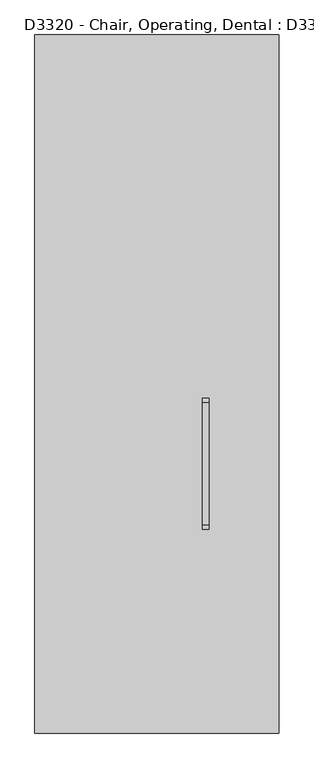
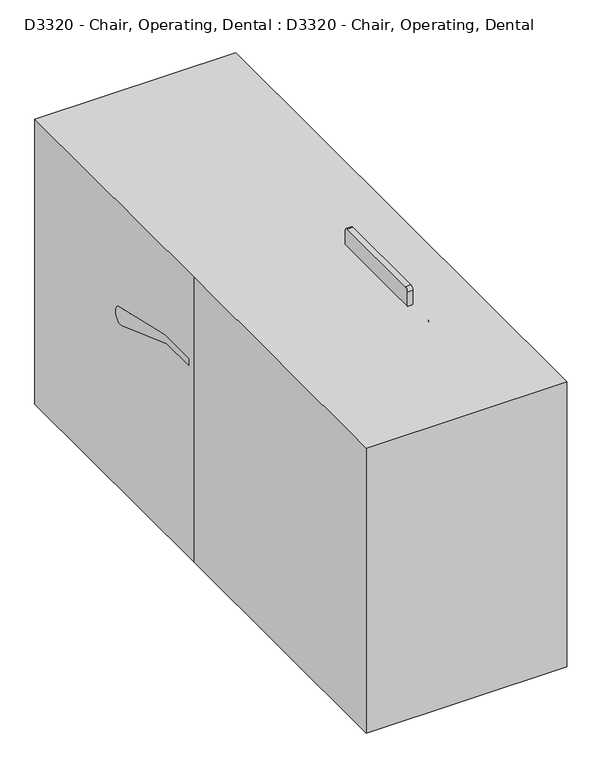
"""IFC4 building model written with IfcOpenShell, lengths in millimetres: proxy geometry, D3320 - Chair, Operating, Dental : D3320 - Chair, Operating, Dental."""

import ifcopenshell
import ifcopenshell.guid

model = None  # the IFC model being written
_history = None  # IfcOwnerHistory: only IFC2X3 demands one
_inside = {}  # id of a spatial element -> (the spatial element, [elements in it])
_under = {}  # id of a project, library or spatial element -> (it, [spatial elements below it])
_declared = {}  # id of a project -> (the project, [libraries it declares])
_typed = {}  # id of a type object -> (the type object, [elements of that type])
_made_of = {}  # id of a material, layer set ... -> (it, [elements and type objects made of it])


def new_model(schema):
    """Start an empty IFC model of exactly this schema.

    Asked for "IFC4X3", IfcOpenShell would pick the latest addendum, in which some entities
    have other attributes; the version numbers below select the first issue.
    IFC2X3 requires an IfcOwnerHistory on every rooted entity: one is made here for all.
    """
    global model, _history
    if schema == "IFC4X3":
        model = ifcopenshell.file(schema_version=(4, 3, 0, 0))
    else:
        model = ifcopenshell.file(schema=schema)
    _inside.clear()
    _under.clear()
    _declared.clear()
    _typed.clear()
    _made_of.clear()
    _history = None
    if model.schema == "IFC2X3":
        org = make("IfcOrganization", Name="unknown")
        user = make(
            "IfcPersonAndOrganization",
            ThePerson=make("IfcPerson", FamilyName="unknown"),
            TheOrganization=org,
        )
        app = make(
            "IfcApplication",
            ApplicationDeveloper=org,
            Version="unknown",
            ApplicationFullName="unknown",
            ApplicationIdentifier="unknown",
        )
        _history = make(
            "IfcOwnerHistory",
            OwningUser=user,
            OwningApplication=app,
            ChangeAction="ADDED",
            CreationDate=0,
        )
    return model


def make(cls, **values):
    """One entity of the class cls with the attributes given. An attribute that is None is left unset."""
    return model.create_entity(
        cls, **{name: value for name, value in values.items() if value is not None}
    )


def rooted(cls, **values):
    """An entity with a GlobalId (a new one), such as an element, a storey or a relation."""
    return make(cls, GlobalId=ifcopenshell.guid.new(), OwnerHistory=_history, **values)


def si_unit(unit_type, name, prefix=None):
    """IfcSIUnit, for example si_unit("LENGTHUNIT", "METRE", prefix="MILLI")."""
    return make("IfcSIUnit", UnitType=unit_type, Prefix=prefix, Name=name)


def assignment(units):
    """IfcUnitAssignment: the units of a project."""
    return None if units is None else make("IfcUnitAssignment", Units=units)


def point(xyz):
    """IfcCartesianPoint."""
    return None if xyz is None else make("IfcCartesianPoint", Coordinates=xyz)


def direction(xyz):
    """IfcDirection."""
    return None if xyz is None else make("IfcDirection", DirectionRatios=xyz)


def frame(location, z_axis=None, x_axis=None):
    """IfcAxis2Placement3D, a coordinate frame: its origin and axes. An axis left out is left unset."""
    return make(
        "IfcAxis2Placement3D",
        Location=point(location),
        Axis=direction(z_axis),
        RefDirection=direction(x_axis),
    )


def frame_2d(location, x_axis=None):
    """IfcAxis2Placement2D, a coordinate frame in the plane: its origin and x axis."""
    return make(
        "IfcAxis2Placement2D", Location=point(location), RefDirection=direction(x_axis)
    )


def origin():
    """The frame at (0, 0, 0) with its axes left unset."""
    return frame((0.0, 0.0, 0.0))


def origin_with_axes():
    """The frame at (0, 0, 0) with the z axis (0, 0, 1) and the x axis (1, 0, 0) written out."""
    return frame((0.0, 0.0, 0.0), z_axis=(0.0, 0.0, 1.0), x_axis=(1.0, 0.0, 0.0))


def place(relative_to, where):
    """IfcLocalPlacement: puts the frame where relative to a parent placement (None: the world)."""
    return make(
        "IfcLocalPlacement", PlacementRelTo=relative_to, RelativePlacement=where
    )


def context(
    kind, dimensions, precision=None, world=None, true_north=None, identifier=None
):
    """IfcGeometricRepresentationContext, for example the 3D "Model" context."""
    return make(
        "IfcGeometricRepresentationContext",
        ContextIdentifier=identifier,
        ContextType=kind,
        CoordinateSpaceDimension=dimensions,
        Precision=precision,
        WorldCoordinateSystem=world,
        TrueNorth=true_north,
    )


def project(units=None, contexts=None):
    """IfcProject with its units and contexts."""
    return rooted(
        "IfcProject",
        Name="project",
        RepresentationContexts=contexts,
        UnitsInContext=assignment(units),
    )


def spatial(cls, under=None, at=None, **own):
    """A site, building, storey or space (cls), placed at a placement, below another one or the project."""
    s = rooted(cls, ObjectPlacement=at, **own)
    if under is not None:
        _under.setdefault(under.id(), (under, []))[1].append(s)
    return s


def polyline(points):
    """IfcPolyline through the points."""
    return make("IfcPolyline", Points=[point(p) for p in points])


def circle_curve(where, radius):
    """IfcCircle in the frame where."""
    return make("IfcCircle", Position=where, Radius=radius)


def ellipse_curve(where, semi_axis1, semi_axis2):
    """IfcEllipse in the frame where."""
    return make(
        "IfcEllipse", Position=where, SemiAxis1=semi_axis1, SemiAxis2=semi_axis2
    )


def trimmed(basis, trim1, trim2, sense, master):
    """IfcTrimmedCurve: the piece of a basis curve between two trims."""
    return make(
        "IfcTrimmedCurve",
        BasisCurve=basis,
        Trim1=trim1,
        Trim2=trim2,
        SenseAgreement=sense,
        MasterRepresentation=master,
    )


def segment(curve, same_sense, transition):
    """IfcCompositeCurveSegment."""
    return make(
        "IfcCompositeCurveSegment",
        Transition=transition,
        SameSense=same_sense,
        ParentCurve=curve,
    )


def composite_curve(segments, self_intersect=None):
    """IfcCompositeCurve: segments joined end to end."""
    return make("IfcCompositeCurve", Segments=segments, SelfIntersect=self_intersect)


def outline(outer, holes=None, kind="AREA"):
    """IfcArbitraryClosedProfileDef: a profile drawn as a closed curve; with holes, ...WithVoids."""
    if holes is None:
        return make("IfcArbitraryClosedProfileDef", ProfileType=kind, OuterCurve=outer)
    return make(
        "IfcArbitraryProfileDefWithVoids",
        ProfileType=kind,
        OuterCurve=outer,
        InnerCurves=holes,
    )


def extrude(swept, where, along, depth):
    """IfcExtrudedAreaSolid: the profile swept, set in the frame where, extruded along a direction by depth."""
    return make(
        "IfcExtrudedAreaSolid",
        SweptArea=swept,
        Position=where,
        ExtrudedDirection=direction(along),
        Depth=depth,
    )


def shape(context_of_items, identifier, shape_type, items):
    """IfcShapeRepresentation: the items that make up one representation, for example the "Body"."""
    return make(
        "IfcShapeRepresentation",
        ContextOfItems=context_of_items,
        RepresentationIdentifier=identifier,
        RepresentationType=shape_type,
        Items=items,
    )


def source(mapping_origin, context_of_items, identifier, shape_type, items):
    """IfcRepresentationMap: a shape defined once, which mapped items show again and again."""
    return make(
        "IfcRepresentationMap",
        MappingOrigin=mapping_origin,
        MappedRepresentation=shape(context_of_items, identifier, shape_type, items),
    )


def transform(
    local_origin,
    x_axis=None,
    y_axis=None,
    z_axis=None,
    scale=None,
    scale2=None,
    scale3=None,
    uniform=True,
):
    """IfcCartesianTransformationOperator3D, or its non-uniform kind. x_axis, y_axis, z_axis: its Axis1, 2, 3."""
    if uniform:
        return make(
            "IfcCartesianTransformationOperator3D",
            Axis1=direction(x_axis),
            Axis2=direction(y_axis),
            LocalOrigin=point(local_origin),
            Scale=scale,
            Axis3=direction(z_axis),
        )
    return make(
        "IfcCartesianTransformationOperator3DnonUniform",
        Axis1=direction(x_axis),
        Axis2=direction(y_axis),
        LocalOrigin=point(local_origin),
        Scale=scale,
        Axis3=direction(z_axis),
        Scale2=scale2,
        Scale3=scale3,
    )


def mapped(mapping_source, mapping_target):
    """IfcMappedItem: shows the shape of a source again, moved by a transform."""
    return make(
        "IfcMappedItem", MappingSource=mapping_source, MappingTarget=mapping_target
    )


def made_of(thing, what):
    """Note that an element or type object is made of a material, layer set ...; save() writes the relation."""
    if what is not None:
        _made_of.setdefault(what.id(), (what, []))[1].append(thing)
    return thing


def element(
    cls,
    number,
    at=None,
    inside=None,
    cuts=None,
    type_object=None,
    material=None,
    context=None,
    identifier="Body",
    shape_type=None,
    held_by="IfcProductDefinitionShape",
    body=None,
    shapes=None,
    **own,
):
    """One element of the class cls, such as IfcWall. Its Tag is "e" and its number.

    at: its placement. inside: the storey or other place that contains it. cuts: it is an
    opening in that element (IfcRelVoidsElement). A single representation is given by context,
    identifier, shape_type and body (its items); several are given by shapes. held_by: the class
    of the entity that holds the representations. save() writes the other relations.
    """
    e = rooted(cls, Tag="e%d" % number, ObjectPlacement=at, **own)
    if body is not None:
        shapes = [shape(context, identifier, shape_type, body)]
    if shapes is not None:
        e.Representation = make(held_by, Representations=shapes)
    if inside is not None:
        _inside.setdefault(inside.id(), (inside, []))[1].append(e)
    if cuts is not None:
        rooted(
            "IfcRelVoidsElement", RelatingBuildingElement=cuts, RelatedOpeningElement=e
        )
    if type_object is not None:
        _typed.setdefault(type_object.id(), (type_object, []))[1].append(e)
    return made_of(e, material)


def aggregate(whole, parts):
    """IfcRelAggregates: a whole, such as a stair, and the parts it consists of."""
    return rooted("IfcRelAggregates", RelatingObject=whole, RelatedObjects=parts)


def save(model, path):
    """Write the relations noted so far, then the file.

    IfcRelAggregates (storeys below a building ...), IfcRelContainedInSpatialStructure (elements
    in a storey), IfcRelDefinesByType, IfcRelAssociatesMaterial and IfcRelDeclares: one each for
    every whole, place, type object, material and project.
    """
    for whole, parts in _under.values():
        aggregate(whole, parts)
    for where, things in _inside.values():
        rooted(
            "IfcRelContainedInSpatialStructure",
            RelatedElements=things,
            RelatingStructure=where,
        )
    for kind, things in _typed.values():
        rooted("IfcRelDefinesByType", RelatedObjects=things, RelatingType=kind)
    for what, things in _made_of.values():
        rooted("IfcRelAssociatesMaterial", RelatedObjects=things, RelatingMaterial=what)
    for by, libraries in _declared.values():
        rooted("IfcRelDeclares", RelatingContext=by, RelatedDefinitions=libraries)
    model.write(path)


def plane_surface(at):
    """IfcPlane: the flat surface through the origin of the frame at, square to its z axis."""
    return make("IfcPlane", Position=at)


def cylinder_surface(at, radius):
    """IfcCylindricalSurface: all points at the distance radius from the z axis of the frame at."""
    return make("IfcCylindricalSurface", Position=at, Radius=radius)


def revolved_surface(curve, axis_point, axis_direction):
    """IfcSurfaceOfRevolution: the curve turned about the line through axis_point along axis_direction."""
    return make(
        "IfcSurfaceOfRevolution",
        SweptCurve=make("IfcArbitraryOpenProfileDef", ProfileType="CURVE", Curve=curve),
        AxisPosition=make("IfcAxis1Placement", Location=point(axis_point), Axis=direction(axis_direction)),
    )


def spline_surface(u_degree, v_degree, points, u_multiplicities, v_multiplicities, u_knots, v_knots, weights=None):
    """IfcBSplineSurfaceWithKnots; with weights, IfcRationalBSplineSurfaceWithKnots. points: one row for each step in u."""
    own = dict(
        UDegree=u_degree,
        VDegree=v_degree,
        ControlPointsList=[[point(p) for p in row] for row in points],
        SurfaceForm="UNSPECIFIED",
        UClosed=False,
        VClosed=False,
        SelfIntersect=False,
        UMultiplicities=u_multiplicities,
        VMultiplicities=v_multiplicities,
        UKnots=u_knots,
        VKnots=v_knots,
        KnotSpec="UNSPECIFIED",
    )
    if weights is None:
        return make("IfcBSplineSurfaceWithKnots", **own)
    return make("IfcRationalBSplineSurfaceWithKnots", WeightsData=weights, **own)


def advanced_brep(points, edges, surfaces, faces):
    """IfcAdvancedBrep: a solid bounded by faces that lie on surfaces and meet in shared edges.

    An edge is (start, end): straight between two places in points (the first is 0);
    or (start, end, curve); or (start, end, curve, False) where it runs against its curve.
    A face is (place in surfaces, loops), or (place, loops, False) where it looks against
    its surface's normal. A loop lists edges by number (the first is 1), with a minus sign
    where the edge is run from its end to its start. The first loop is the outer one.
    """
    corners = [point(p) for p in points]
    vertices = [make("IfcVertexPoint", VertexGeometry=c) for c in corners]
    made = []
    for start, end, *more in edges:
        made.append(
            make(
                "IfcEdgeCurve",
                EdgeStart=vertices[start],
                EdgeEnd=vertices[end],
                EdgeGeometry=more[0] if more else make("IfcPolyline", Points=[corners[start], corners[end]]),
                SameSense=more[1] if len(more) > 1 else True,
            )
        )
    hull = []
    for where, loops, *sense in faces:
        bounds = []
        for j, loop in enumerate(loops):
            ring = [make("IfcOrientedEdge", EdgeElement=made[abs(k) - 1], Orientation=k > 0) for k in loop]
            bounds.append(
                make(
                    "IfcFaceOuterBound" if j == 0 else "IfcFaceBound",
                    Bound=make("IfcEdgeLoop", EdgeList=ring),
                    Orientation=True,
                )
            )
        hull.append(make("IfcAdvancedFace", Bounds=bounds, FaceSurface=surfaces[where], SameSense=sense[0] if sense else True))
    return make("IfcAdvancedBrep", Outer=make("IfcClosedShell", CfsFaces=hull))


def d3320_chair_operating_dental_d3320_chair_operating_dental_678bfee4(model_context):
    return source(origin(), model_context, "Body", "SolidModel", [
        advanced_brep(
        [(330.2, -282.0868489, 807.4979758), (330.2, -282.0868489, 845.5979758), (330.2, -212.2368489, 877.3479758), (330.2, -250.3368489, 877.3479758)],
        [
            (0, 1, circle_curve(frame((330.2, -282.0868489, 826.5479758), z_axis=(0.0, -1.0, 0.0), x_axis=(0.0, 0.0, 1.0)), 19.05)),
            (1, 0, circle_curve(frame((330.2, -282.0868489, 826.5479758), z_axis=(0.0, -1.0, 0.0), x_axis=(0.0, 0.0, 1.0)), 19.05)),
            (2, 3, circle_curve(frame((330.2, -231.2868489, 877.3479758), z_axis=(0.0, 0.0, 1.0), x_axis=(0.0, -1.0, 0.0)), 19.05)),
            (3, 2, circle_curve(frame((330.2, -231.2868489, 877.3479758), z_axis=(0.0, 0.0, 1.0), x_axis=(0.0, -1.0, 0.0)), 19.05)),
            (3, 1, circle_curve(frame((330.2, -282.0868489, 877.3479758), z_axis=(-1.0, 0.0, 0.0), x_axis=(0.0, 0.0, -1.0)), 31.75)),
            (0, 2, circle_curve(frame((330.2, -282.0868489, 877.3479758), z_axis=(1.0, 0.0, 0.0), x_axis=(0.0, 0.0, -1.0)), 69.85)),
        ],
        [
            plane_surface(frame((330.2, -282.0868489, 826.5479758), z_axis=(0.0, -1.0, 0.0), x_axis=(1.0, 0.0, 0.0))),
            plane_surface(frame((330.2, -231.2868489, 877.3479758), z_axis=(0.0, 0.0, 1.0), x_axis=(1.0, 0.0, 0.0))),
            revolved_surface(trimmed(ellipse_curve(frame((330.2, -282.0868489, 826.5479758), z_axis=(0.0, -1.0, 0.0), x_axis=(0.0, 0.0, 1.0)), 19.05, 19.05), [point((330.2, -282.0868489, 807.4979758))], [point((330.2, -282.0868489, 845.5979758))], True, "CARTESIAN"), (330.2, -282.0868489, 877.3479758), (1.0, 0.0, 0.0)),
            revolved_surface(trimmed(ellipse_curve(frame((330.2, -282.0868489, 826.5479758), z_axis=(0.0, -1.0, 0.0), x_axis=(0.0, 0.0, 1.0)), 19.05, 19.05), [point((330.2, -282.0868489, 845.5979758))], [point((330.2, -282.0868489, 807.4979758))], True, "CARTESIAN"), (330.2, -282.0868489, 877.3479758), (1.0, 0.0, 0.0)),
        ],
        [
            (0, [[1, 2]]),
            (1, [[3, 4]]),
            (2, [[5, -1, 6, -4]]),
            (3, [[-6, -2, -5, -3]]),
        ],
    ),
        extrude(outline(composite_curve([segment(trimmed(circle_curve(frame_2d((826.5479758, 330.2)), 19.05), [point((807.4979758, 330.2))], [point((845.5979758, 330.2))], False, "CARTESIAN"), True, "CONTINUOUS"), segment(trimmed(circle_curve(frame_2d((826.5479758, 330.2)), 19.05), [point((845.5979758, 330.2))], [point((807.4979758, 330.2))], False, "CARTESIAN"), True, "CONTINUOUS")], self_intersect=False)), frame((0.0, -629.7082464, 0.0), z_axis=(0.0, 1.0, 0.0), x_axis=(0.0, 0.0, 1.0)), (0.0, 0.0, 1.0), 347.6213974),
        advanced_brep(
        [(330.2, -629.7082464, 845.5979758), (330.2, -629.7082464, 807.4979758), (330.2, -699.5582464, 775.7479758), (330.2, -661.4582464, 775.7479758)],
        [
            (0, 1, circle_curve(frame((330.2, -629.7082464, 826.5479758), z_axis=(0.0, 1.0, 0.0), x_axis=(0.0, 0.0, -1.0)), 19.05)),
            (1, 0, circle_curve(frame((330.2, -629.7082464, 826.5479758), z_axis=(0.0, 1.0, 0.0), x_axis=(0.0, 0.0, -1.0)), 19.05)),
            (2, 3, circle_curve(frame((330.2, -680.5082464, 775.7479758), z_axis=(0.0, 0.0, -1.0), x_axis=(0.0, 1.0, 0.0)), 19.05)),
            (3, 2, circle_curve(frame((330.2, -680.5082464, 775.7479758), z_axis=(0.0, 0.0, -1.0), x_axis=(0.0, 1.0, 0.0)), 19.05)),
            (3, 1, circle_curve(frame((330.2, -629.7082464, 775.7479758), z_axis=(-1.0, 0.0, 0.0), x_axis=(0.0, 0.0, 1.0)), 31.75)),
            (0, 2, circle_curve(frame((330.2, -629.7082464, 775.7479758), z_axis=(1.0, 0.0, 0.0), x_axis=(0.0, 0.0, 1.0)), 69.85)),
        ],
        [
            plane_surface(frame((330.2, -629.7082464, 826.5479758), z_axis=(0.0, 1.0, 0.0), x_axis=(1.0, 0.0, 0.0))),
            plane_surface(frame((330.2, -680.5082464, 775.7479758), z_axis=(0.0, 0.0, -1.0), x_axis=(1.0, 0.0, 0.0))),
            revolved_surface(trimmed(ellipse_curve(frame((330.2, -629.7082464, 826.5479758), z_axis=(0.0, 1.0, 0.0), x_axis=(0.0, 0.0, -1.0)), 19.05, 19.05), [point((330.2, -629.7082464, 845.5979758))], [point((330.2, -629.7082464, 807.4979758))], True, "CARTESIAN"), (330.2, -629.7082464, 775.7479758), (1.0, 0.0, 0.0)),
            revolved_surface(trimmed(ellipse_curve(frame((330.2, -629.7082464, 826.5479758), z_axis=(0.0, 1.0, 0.0), x_axis=(0.0, 0.0, -1.0)), 19.05, 19.05), [point((330.2, -629.7082464, 807.4979758))], [point((330.2, -629.7082464, 845.5979758))], True, "CARTESIAN"), (330.2, -629.7082464, 775.7479758), (1.0, 0.0, 0.0)),
        ],
        [
            (0, [[1, 2]]),
            (1, [[3, 4]]),
            (2, [[5, -1, 6, -4]]),
            (3, [[-6, -2, -5, -3]]),
        ],
    ),
        extrude(outline(composite_curve([segment(polyline([(-54.312137, 904.4198133), (-409.912137, 904.4198133)]), True, "CONTINUOUS"), segment(trimmed(circle_curve(frame_2d((-409.912137, 917.1198133)), 12.7), [point((-409.912137, 904.4198133))], [point((-422.612137, 917.1198133))], False, "CARTESIAN"), True, "CONTINUOUS"), segment(polyline([(-422.612137, 917.1198133), (-422.612137, 1120.3198133)]), True, "CONTINUOUS"), segment(trimmed(circle_curve(frame_2d((-409.912137, 1120.3198133)), 12.7), [point((-422.612137, 1120.3198133))], [point((-409.912137, 1133.0198133))], False, "CARTESIAN"), True, "CONTINUOUS"), segment(polyline([(-409.912137, 1133.0198133), (-54.312137, 1133.0198133)]), True, "CONTINUOUS"), segment(trimmed(circle_curve(frame_2d((-54.312137, 1120.3198133)), 12.7), [point((-54.312137, 1133.0198133))], [point((-41.612137, 1120.3198133))], False, "CARTESIAN"), True, "CONTINUOUS"), segment(polyline([(-41.612137, 1120.3198133), (-41.612137, 917.1198133)]), True, "CONTINUOUS"), segment(trimmed(circle_curve(frame_2d((-54.312137, 917.1198133)), 12.7), [point((-41.612137, 917.1198133))], [point((-54.312137, 904.4198133))], False, "CARTESIAN"), True, "CONTINUOUS")], self_intersect=False)), frame((133.35, 0.0, 0.0), z_axis=(1.0, 0.0, 0.0), x_axis=(0.0, 1.0, 0.0)), (0.0, 0.0, 1.0), 19.05),
        advanced_brep(
        [(152.4, -231.2868489, 909.123847), (152.4, -231.2868489, 947.223847), (279.4, -231.2868489, 947.223847), (279.4, -231.2868489, 909.123847), (311.15, -231.2868489, 877.373847), (349.25, -231.2868489, 877.373847)],
        [
            (0, 1, circle_curve(frame((152.4, -231.2868489, 928.173847), z_axis=(-1.0, 0.0, 0.0), x_axis=(0.0, 0.0, 1.0)), 19.05)),
            (1, 0, circle_curve(frame((152.4, -231.2868489, 928.173847), z_axis=(-1.0, 0.0, 0.0), x_axis=(0.0, 0.0, 1.0)), 19.05)),
            (1, 2),
            (2, 3, circle_curve(frame((279.4, -231.2868489, 928.173847), z_axis=(-1.0, 0.0, 0.0), x_axis=(0.0, 0.0, 1.0)), 19.05)),
            (3, 0),
            (3, 2, circle_curve(frame((279.4, -231.2868489, 928.173847), z_axis=(-1.0, 0.0, 0.0), x_axis=(0.0, 0.0, 1.0)), 19.05)),
            (4, 5, circle_curve(frame((330.2, -231.2868489, 877.373847), z_axis=(0.0, 0.0, -1.0), x_axis=(1.0, 0.0, 0.0)), 19.05)),
            (5, 4, circle_curve(frame((330.2, -231.2868489, 877.373847), z_axis=(0.0, 0.0, -1.0), x_axis=(1.0, 0.0, 0.0)), 19.05)),
            (4, 3, circle_curve(frame((279.4, -231.2868489, 877.373847), z_axis=(0.0, -1.0, 0.0), x_axis=(0.0, 0.0, 1.0)), 31.75)),
            (2, 5, circle_curve(frame((279.4, -231.2868489, 877.373847), z_axis=(0.0, 1.0, 0.0), x_axis=(0.0, 0.0, 1.0)), 69.85)),
        ],
        [
            plane_surface(frame((152.4, -231.2868489, 928.173847), z_axis=(-1.0, 0.0, 0.0), x_axis=(0.0, -1.0, 0.0))),
            cylinder_surface(frame((152.4, -231.2868489, 928.173847), z_axis=(-1.0, 0.0, 0.0), x_axis=(0.0, 0.0, 1.0)), 19.05),
            plane_surface(frame((330.2, -231.2868489, 877.373847), z_axis=(0.0, 0.0, -1.0), x_axis=(0.0, -1.0, 0.0))),
            revolved_surface(trimmed(ellipse_curve(frame((279.4, -231.2868489, 928.173847), z_axis=(-1.0, 0.0, 0.0), x_axis=(0.0, 0.0, 1.0)), 19.05, 19.05), [point((279.4, -231.2868489, 947.223847))], [point((279.4, -231.2868489, 909.123847))], True, "CARTESIAN"), (279.4, -231.2868489, 877.373847), (0.0, 1.0, 0.0)),
            revolved_surface(trimmed(ellipse_curve(frame((279.4, -231.2868489, 928.173847), z_axis=(-1.0, 0.0, 0.0), x_axis=(0.0, 0.0, 1.0)), 19.05, 19.05), [point((279.4, -231.2868489, 909.123847))], [point((279.4, -231.2868489, 947.223847))], True, "CARTESIAN"), (279.4, -231.2868489, 877.373847), (0.0, 1.0, 0.0)),
        ],
        [
            (0, [[1, 2]]),
            (1, [[-2, 3, 4, 5]]),
            (1, [[-1, -5, 6, -3]]),
            (2, [[7, 8]]),
            (3, [[9, -4, 10, -7]]),
            (4, [[-10, -6, -9, -8]]),
        ],
    ),
        advanced_brep(
        [(152.4, -680.5082464, 147.0979758), (152.4, -680.5082464, 185.1979758), (279.4, -680.5082464, 147.0979758), (279.4, -680.5082464, 185.1979758), (349.25, -680.5082464, 216.9479758), (311.15, -680.5082464, 216.9479758)],
        [
            (0, 1, circle_curve(frame((152.4, -680.5082464, 166.1479758), z_axis=(-1.0, 0.0, 0.0), x_axis=(0.0, 0.0, 1.0)), 19.05)),
            (1, 0, circle_curve(frame((152.4, -680.5082464, 166.1479758), z_axis=(-1.0, 0.0, 0.0), x_axis=(0.0, 0.0, 1.0)), 19.05)),
            (0, 2),
            (2, 3, circle_curve(frame((279.4, -680.5082464, 166.1479758), z_axis=(-1.0, 0.0, 0.0), x_axis=(0.0, 0.0, 1.0)), 19.05)),
            (3, 1),
            (3, 2, circle_curve(frame((279.4, -680.5082464, 166.1479758), z_axis=(-1.0, 0.0, 0.0), x_axis=(0.0, 0.0, 1.0)), 19.05)),
            (4, 5, circle_curve(frame((330.2, -680.5082464, 216.9479758), z_axis=(0.0, 0.0, 1.0), x_axis=(-1.0, 0.0, 0.0)), 19.05)),
            (5, 4, circle_curve(frame((330.2, -680.5082464, 216.9479758), z_axis=(0.0, 0.0, 1.0), x_axis=(-1.0, 0.0, 0.0)), 19.05)),
            (5, 3, circle_curve(frame((279.4, -680.5082464, 216.9479758), z_axis=(0.0, 1.0, 0.0), x_axis=(0.0, 0.0, -1.0)), 31.75)),
            (2, 4, circle_curve(frame((279.4, -680.5082464, 216.9479758), z_axis=(0.0, -1.0, 0.0), x_axis=(0.0, 0.0, -1.0)), 69.85)),
        ],
        [
            plane_surface(frame((152.4, -680.5082464, 166.1479758), z_axis=(-1.0, 0.0, 0.0), x_axis=(0.0, -1.0, 0.0))),
            cylinder_surface(frame((152.4, -680.5082464, 166.1479758), z_axis=(-1.0, 0.0, 0.0), x_axis=(0.0, 0.0, 1.0)), 19.05),
            plane_surface(frame((330.2, -680.5082464, 216.9479758), z_axis=(0.0, 0.0, 1.0), x_axis=(0.0, -1.0, 0.0))),
            revolved_surface(trimmed(ellipse_curve(frame((279.4, -680.5082464, 166.1479758), z_axis=(-1.0, 0.0, 0.0), x_axis=(0.0, 0.0, 1.0)), 19.05, 19.05), [point((279.4, -680.5082464, 147.0979758))], [point((279.4, -680.5082464, 185.1979758))], True, "CARTESIAN"), (279.4, -680.5082464, 216.9479758), (0.0, -1.0, 0.0)),
            revolved_surface(trimmed(ellipse_curve(frame((279.4, -680.5082464, 166.1479758), z_axis=(-1.0, 0.0, 0.0), x_axis=(0.0, 0.0, 1.0)), 19.05, 19.05), [point((279.4, -680.5082464, 185.1979758))], [point((279.4, -680.5082464, 147.0979758))], True, "CARTESIAN"), (279.4, -680.5082464, 216.9479758), (0.0, -1.0, 0.0)),
        ],
        [
            (0, [[1, 2]]),
            (1, [[-1, 3, 4, 5]]),
            (1, [[-2, -5, 6, -3]]),
            (2, [[7, 8]]),
            (3, [[9, -4, 10, -8]]),
            (4, [[-10, -6, -9, -7]]),
        ],
    ),
        extrude(outline(composite_curve([segment(trimmed(circle_curve(frame_2d((493.8256126, 645.6714008)), 19.05), [point((474.7756126, 645.6714008))], [point((512.8756126, 645.6714008))], False, "CARTESIAN"), True, "CONTINUOUS"), segment(trimmed(circle_curve(frame_2d((493.8256126, 645.6714008)), 19.05), [point((512.8756126, 645.6714008))], [point((474.7756126, 645.6714008))], False, "CARTESIAN"), True, "CONTINUOUS")], self_intersect=False)), frame((-306.1189765, 0.0, 0.0), z_axis=(1.0, 0.0, 0.0), x_axis=(0.0, 1.0, 0.0)), (0.0, 0.0, 1.0), 610.9189765),
        extrude(outline(composite_curve([segment(trimmed(circle_curve(frame_2d((330.2, -680.5082464)), 19.05), [point((349.25, -680.5082464))], [point((311.15, -680.5082464))], False, "CARTESIAN"), True, "CONTINUOUS"), segment(trimmed(circle_curve(frame_2d((330.2, -680.5082464)), 19.05), [point((311.15, -680.5082464))], [point((349.25, -680.5082464))], False, "CARTESIAN"), True, "CONTINUOUS")], self_intersect=False)), frame((0.0, 0.0, 216.9479758), z_axis=(0.0, 0.0, 1.0), x_axis=(1.0, 0.0, 0.0)), (0.0, 0.0, 1.0), 558.8),
        extrude(outline(composite_curve([segment(trimmed(circle_curve(frame_2d((208.2843617, -50.8)), 50.8), [point((208.2843617, 0.0))], [point((243.3133982, -14.0086069))], False, "CARTESIAN"), True, "CONTINUOUS"), segment(polyline([(243.3133982, -14.0086069), (332.2133982, -167.9879237)]), True, "CONTINUOUS"), segment(trimmed(circle_curve(frame_2d((16.6967808, -350.1515277)), 364.327208), [point((332.2133982, -167.9879237))], [point((381.0, -345.9707394))], False, "CARTESIAN"), True, "CONTINUOUS"), segment(polyline([(381.0, -345.9707394), (381.0, -422.1707394)]), True, "CONTINUOUS"), segment(trimmed(circle_curve(frame_2d((182.0559291, -422.1707394)), 198.9440709), [point((381.0, -422.1707394))], [point((309.9347128, -574.5707394))], False, "CARTESIAN"), True, "CONTINUOUS"), segment(polyline([(309.9347128, -574.5707394), (-50.8, -574.5707394)]), True, "CONTINUOUS"), segment(trimmed(circle_curve(frame_2d((22.4448791, -442.6982999)), 150.8481111), [point((-50.8, -574.5707394))], [point((-127.0, -422.1707394))], False, "CARTESIAN"), True, "CONTINUOUS"), segment(polyline([(-127.0, -422.1707394), (-127.0, -345.9707394)]), True, "CONTINUOUS"), segment(trimmed(circle_curve(frame_2d((237.3032191, -350.1515277)), 364.327208), [point((-127.0, -345.9707394))], [point((-78.2133983, -167.9879237))], False, "CARTESIAN"), True, "CONTINUOUS"), segment(polyline([(-78.2133983, -167.9879237), (10.6866017, -14.0086069)]), True, "CONTINUOUS"), segment(trimmed(circle_curve(frame_2d((45.7156382, -50.8)), 50.8), [point((10.6866017, -14.0086069))], [point((45.7156382, 0.0))], False, "CARTESIAN"), True, "CONTINUOUS"), segment(polyline([(45.7156382, 0.0), (208.2843617, 0.0)]), True, "CONTINUOUS")], self_intersect=False)), frame((-129.5673564, 864.322553, 876.3857997), z_axis=(0.0, -0.6156614753256581, 0.7880107536067222), x_axis=(1.0, 0.0, 0.0)), (0.0, 0.0, 1.0), 25.4),
        extrude(outline(composite_curve([segment(trimmed(circle_curve(frame_2d((208.2843617, -50.8)), 50.8), [point((208.2843617, 0.0))], [point((243.3133982, -14.0086069))], False, "CARTESIAN"), True, "CONTINUOUS"), segment(polyline([(243.3133982, -14.0086069), (332.2133982, -167.9879237)]), True, "CONTINUOUS"), segment(trimmed(circle_curve(frame_2d((16.6967808, -350.1515277)), 364.327208), [point((332.2133982, -167.9879237))], [point((381.0, -345.9707394))], False, "CARTESIAN"), True, "CONTINUOUS"), segment(polyline([(381.0, -345.9707394), (381.0, -422.1707394)]), True, "CONTINUOUS"), segment(trimmed(circle_curve(frame_2d((182.0559291, -422.1707394)), 198.9440709), [point((381.0, -422.1707394))], [point((309.9347128, -574.5707394))], False, "CARTESIAN"), True, "CONTINUOUS"), segment(polyline([(309.9347128, -574.5707394), (-50.8, -574.5707394)]), True, "CONTINUOUS"), segment(trimmed(circle_curve(frame_2d((22.4448791, -442.6982998)), 150.8481111), [point((-50.8, -574.5707394))], [point((-127.0, -422.1707394))], False, "CARTESIAN"), True, "CONTINUOUS"), segment(polyline([(-127.0, -422.1707394), (-127.0, -345.9707394)]), True, "CONTINUOUS"), segment(trimmed(circle_curve(frame_2d((237.3032191, -350.1515277)), 364.327208), [point((-127.0, -345.9707394))], [point((-78.2133983, -167.9879237))], False, "CARTESIAN"), True, "CONTINUOUS"), segment(polyline([(-78.2133983, -167.9879237), (10.6866017, -14.0086069)]), True, "CONTINUOUS"), segment(trimmed(circle_curve(frame_2d((45.7156382, -50.8)), 50.8), [point((10.6866017, -14.0086069))], [point((45.7156382, 0.0))], False, "CARTESIAN"), True, "CONTINUOUS"), segment(polyline([(45.7156382, 0.0), (208.2843617, 0.0)]), True, "CONTINUOUS")], self_intersect=False)), frame((-129.5673564, 848.6847515, 896.4012729), z_axis=(0.0, -0.6156614753256581, 0.7880107536067222), x_axis=(1.0, 0.0, 0.0)), (0.0, 0.0, 1.0), 50.8),
        extrude(outline(composite_curve([segment(trimmed(circle_curve(frame_2d((489.7654805, 647.772225)), 31.75), [point((504.1673656, 676.0679527))], [point((478.9625427, 617.9165884))], False, "CARTESIAN"), True, "CONTINUOUS"), segment(polyline([(478.9625427, 617.9165884), (206.8538697, 716.3761557), (73.5038697, 716.3761557), (73.5038697, 741.7761557), (219.5538697, 741.7761557), (504.1673656, 676.0679527)]), True, "CONTINUOUS")], self_intersect=False)), frame((304.8, 0.0, 0.0), z_axis=(1.0, 0.0, 0.0), x_axis=(0.0, 1.0, 0.0)), (0.0, 0.0, 1.0), 50.8),
        extrude(outline(composite_curve([segment(trimmed(circle_curve(frame_2d((489.7654805, 647.772225)), 31.75), [point((504.1673656, 676.0679527))], [point((478.9625427, 617.9165884))], False, "CARTESIAN"), True, "CONTINUOUS"), segment(polyline([(478.9625427, 617.9165884), (206.8538697, 716.3761557), (73.5038697, 716.3761557), (73.5038697, 741.7761557), (219.5538697, 741.7761557), (504.1673656, 676.0679527)]), True, "CONTINUOUS")], self_intersect=False)), frame((-355.6, 0.0, 0.0), z_axis=(1.0, 0.0, 0.0), x_axis=(0.0, 1.0, 0.0)), (0.0, 0.0, 1.0), 50.8),
        extrude(outline(polyline([(310.7877426, 480.8103013), (395.9168302, 542.6602038), (411.5546317, 522.6447306), (310.7877426, 449.4333003), (310.7877426, 480.8103013)])), frame((-50.8, 0.0, 0.0), z_axis=(1.0, 0.0, 0.0), x_axis=(0.0, 1.0, 0.0)), (0.0, 0.0, 1.0), 101.6),
        extrude(outline(polyline([(0.0, -12.7000001), (0.0, 0.0), (50.8, 0.0), (50.8, -12.7000001), (0.0, -12.7000001)])), frame((25.4, 864.322553, 876.3857997), z_axis=(0.0, -0.6156614753256595, 0.788010753606721), x_axis=(-1.0, 0.0, 0.0)), (0.0, 0.0, 1.0), 25.4),
        extrude(outline(composite_curve([segment(trimmed(circle_curve(frame_2d((101.6, -50.8)), 50.8), [point((101.6, 0.0))], [point((152.4, -50.8))], False, "CARTESIAN"), True, "CONTINUOUS"), segment(polyline([(152.4, -50.8), (152.4, -101.6)]), True, "CONTINUOUS"), segment(trimmed(circle_curve(frame_2d((101.6, -101.6)), 50.8), [point((152.4, -101.6))], [point((101.6, -152.3999999))], False, "CARTESIAN"), True, "CONTINUOUS"), segment(polyline([(101.6, -152.3999999), (50.8, -152.3999999)]), True, "CONTINUOUS"), segment(trimmed(circle_curve(frame_2d((50.8, -101.6)), 50.8), [point((50.8, -152.3999999))], [point((0.0, -101.6))], False, "CARTESIAN"), True, "CONTINUOUS"), segment(polyline([(0.0, -101.6), (0.0, -50.8)]), True, "CONTINUOUS"), segment(trimmed(circle_curve(frame_2d((50.8, -50.8)), 50.8), [point((0.0, -50.8))], [point((50.8, 0.0))], False, "CARTESIAN"), True, "CONTINUOUS"), segment(polyline([(50.8, 0.0), (101.6, 0.0)]), True, "CONTINUOUS")], self_intersect=False)), frame((-76.2, 994.4231284, 978.0315093), z_axis=(0.0, -0.6156614753256581, 0.7880107536067222), x_axis=(1.0, 0.0, 0.0)), (0.0, 0.0, 1.0), 25.4),
        extrude(outline(composite_curve([segment(trimmed(circle_curve(frame_2d((101.6, -50.8)), 50.8), [point((101.6, 0.0))], [point((152.4, -50.8))], False, "CARTESIAN"), True, "CONTINUOUS"), segment(polyline([(152.4, -50.8), (152.4, -101.6)]), True, "CONTINUOUS"), segment(trimmed(circle_curve(frame_2d((101.6, -101.6)), 50.8), [point((152.4, -101.6))], [point((101.6, -152.4))], False, "CARTESIAN"), True, "CONTINUOUS"), segment(polyline([(101.6, -152.4), (50.8, -152.4)]), True, "CONTINUOUS"), segment(trimmed(circle_curve(frame_2d((50.8, -101.6)), 50.8), [point((50.8, -152.4))], [point((0.0, -101.6))], False, "CARTESIAN"), True, "CONTINUOUS"), segment(polyline([(0.0, -101.6), (0.0, -50.8)]), True, "CONTINUOUS"), segment(trimmed(circle_curve(frame_2d((50.8, -50.8)), 50.8), [point((0.0, -50.8))], [point((50.8, 0.0))], False, "CARTESIAN"), True, "CONTINUOUS"), segment(polyline([(50.8, 0.0), (101.6, 0.0)]), True, "CONTINUOUS")], self_intersect=False)), frame((-76.2, 978.7853269, 998.0469825), z_axis=(0.0, -0.6156614753256581, 0.7880107536067222), x_axis=(1.0, 0.0, 0.0)), (0.0, 0.0, 1.0), 50.8),
        extrude(outline(polyline([(336.1877426, 524.8043918), (310.7877426, 480.8103013), (-272.8576262, 594.2594685), (-295.1268804, 639.918206), (336.1877426, 524.8043918)])), frame((-304.8, 0.0, 0.0), z_axis=(1.0, 0.0, 0.0), x_axis=(0.0, 1.0, 0.0)), (0.0, 0.0, 1.0), 609.6),
        extrude(outline(composite_curve([segment(polyline([(598.2189765, 0.0), (532.7462193, -533.2328165)]), True, "CONTINUOUS"), segment(trimmed(circle_curve(frame_2d((274.2361884, -526.7589345)), 258.5910811), [point((532.7462193, -533.2328165))], [point((338.8867287, -777.137957))], False, "CARTESIAN"), True, "CONTINUOUS"), segment(polyline([(338.8867287, -777.137957), (245.3132713, -777.137957)]), True, "CONTINUOUS"), segment(trimmed(circle_curve(frame_2d((309.9638116, -526.7589345)), 258.5910811), [point((245.3132713, -777.137957))], [point((51.4537807, -533.2328165))], False, "CARTESIAN"), True, "CONTINUOUS"), segment(polyline([(51.4537807, -533.2328165), (-14.0189765, 0.0), (598.2189765, 0.0)]), True, "CONTINUOUS")], self_intersect=False)), frame((-292.1, -283.3586332, 589.1377851), z_axis=(0.0, -0.4383711467890792, 0.8987940462991661), x_axis=(1.0, 0.0, 0.0)), (0.0, 0.0, 1.0), 50.8),
        extrude(outline(composite_curve([segment(polyline([(-272.8576262, 594.2594685), (310.7877426, 480.8103013), (310.7877426, 452.8366621)]), True, "CONTINUOUS"), segment(trimmed(circle_curve(frame_2d((259.9877426, 452.8366621)), 50.8), [point((310.7877426, 452.8366621))], [point((259.9877426, 402.0366621))], False, "CARTESIAN"), True, "CONTINUOUS"), segment(polyline([(259.9877426, 402.0366621), (90.373422, 402.0366621)]), True, "CONTINUOUS"), segment(trimmed(circle_curve(frame_2d((90.373422, 452.8366621)), 50.8), [point((90.373422, 402.0366621))], [point((74.4163817, 404.6079065))], False, "CARTESIAN"), True, "CONTINUOUS"), segment(polyline([(74.4163817, 404.6079065), (-364.1751013, 549.7209599), (-272.8576262, 594.2594685)]), True, "CONTINUOUS")], self_intersect=False)), frame((-254.0, 0.0, 0.0), z_axis=(1.0, 0.0, 0.0), x_axis=(0.0, 1.0, 0.0)), (0.0, 0.0, 1.0), 508.0),
        extrude(outline(composite_curve([segment(trimmed(circle_curve(frame_2d((154.8195441, 313.1366621)), 80.8223051), [point((235.6418492, 313.1366621))], [point((154.8195441, 232.314357))], False, "CARTESIAN"), True, "CONTINUOUS"), segment(polyline([(154.8195441, 232.314357), (135.7695441, 232.314357)]), True, "CONTINUOUS"), segment(trimmed(circle_curve(frame_2d((135.7695441, 411.5922374)), 179.2778804), [point((135.7695441, 232.314357))], [point((-40.7847024, 442.7235146))], False, "CARTESIAN"), True, "CONTINUOUS"), segment(polyline([(-40.7847024, 442.7235146), (74.4163817, 404.6079065)]), True, "CONTINUOUS"), segment(trimmed(circle_curve(frame_2d((90.373422, 452.8366621)), 50.8), [point((74.4163817, 404.6079065))], [point((88.8729292, 402.0588271))], True, "CARTESIAN"), True, "CONTINUOUS"), segment(polyline([(88.8729292, 402.0588271), (235.6418492, 402.0588271), (235.6418492, 313.1366621)]), True, "CONTINUOUS")], self_intersect=False)), frame((-152.4, 0.0, 0.0), z_axis=(1.0, 0.0, 0.0), x_axis=(0.0, 1.0, 0.0)), (0.0, 0.0, 1.0), 304.8),
        extrude(outline(composite_curve([segment(polyline([(-203.6480621, 317.5988676), (-34.8553722, 356.5677306)]), True, "CONTINUOUS"), segment(trimmed(circle_curve(frame_2d((135.7695441, 411.5922374)), 179.2778804), [point((-34.8553722, 356.5677306))], [point((43.7175474, 257.7514485))], True, "CARTESIAN"), True, "CONTINUOUS"), segment(polyline([(43.7175474, 257.7514485), (-123.4829714, 209.8074713)]), True, "CONTINUOUS"), segment(trimmed(circle_curve(frame_2d((-381.5323002, 101.6)), 279.8183571), [point((-123.4829714, 209.8074713))], [point((-203.6480621, 317.5988676))], True, "CARTESIAN"), True, "CONTINUOUS")], self_intersect=False)), frame((-101.6, 0.0, 0.0), z_axis=(1.0, 0.0, 0.0), x_axis=(0.0, 1.0, 0.0)), (0.0, 0.0, 1.0), 203.2),
        extrude(outline(composite_curve([segment(polyline([(-101.7139431, 101.6), (-101.7139431, 50.8), (-635.0, 50.8), (-635.0, 0.0), (-849.2666885, 0.0), (-849.2666885, 50.8)]), True, "CONTINUOUS"), segment(trimmed(circle_curve(frame_2d((-318.519921, -255.6267891)), 612.8535782), [point((-849.2666885, 50.8))], [point((-318.519921, 357.2267891))], False, "CARTESIAN"), True, "CONTINUOUS"), segment(polyline([(-318.519921, 357.2267891), (-267.719921, 357.2267891)]), True, "CONTINUOUS"), segment(trimmed(circle_curve(frame_2d((-381.5323002, 101.6)), 279.8183571), [point((-267.719921, 357.2267891))], [point((-101.7139431, 101.6))], False, "CARTESIAN"), True, "CONTINUOUS")], self_intersect=False)), frame((-152.4, 0.0, 0.0), z_axis=(1.0, 0.0, 0.0), x_axis=(0.0, 1.0, 0.0)), (0.0, 0.0, 1.0), 304.8),
        extrude(outline(polyline([(368.7784529, 132.1863323), (418.5919512, 122.2236326), (418.5919512, 115.8736326), (368.7784529, 125.8363323), (368.7784529, 132.1863323)])), frame((-48.8615302, 0.0, 0.0), z_axis=(1.0, 0.0, 0.0), x_axis=(0.0, 1.0, 0.0)), (0.0, 0.0, 1.0), 36.3232839),
        extrude(outline(polyline([(368.7784529, 132.1863323), (418.5919512, 122.2236326), (418.5919512, 115.8736326), (368.7784529, 125.8363323), (368.7784529, 132.1863323)])), frame((12.5382463, 0.0, 0.0), z_axis=(1.0, 0.0, 0.0), x_axis=(0.0, 1.0, 0.0)), (0.0, 0.0, 1.0), 36.3232839),
        extrude(outline(polyline([(426.4601145, 101.6), (356.2918492, 101.6), (356.2918492, 128.3336531), (426.4601145, 114.3), (426.4601145, 101.6)])), frame((-63.5, 0.0, 0.0), z_axis=(1.0, 0.0, 0.0), x_axis=(0.0, 1.0, 0.0)), (0.0, 0.0, 1.0), 127.0),
        advanced_brep(
        [(101.6, 392.0977021, 101.6), (-101.6, 392.0977021, 101.6), (127.0, 392.0977021, 50.8), (-127.0, 392.0977021, 50.8)],
        [
            (0, 1, ellipse_curve(frame((0.0, 392.0977021, 101.6), z_axis=(0.0, 0.0, 1.0), x_axis=(-1.0, 0.0, 0.0)), 101.6, 50.8)),
            (1, 0, ellipse_curve(frame((0.0, 392.0977021, 101.6), z_axis=(0.0, 0.0, 1.0), x_axis=(-1.0, 0.0, 0.0)), 101.6, 50.8)),
            (2, 3, ellipse_curve(frame((0.0, 392.0977021, 50.8), z_axis=(0.0, 0.0, -1.0), x_axis=(-1.0, 0.0, 0.0)), 127.0, 63.5)),
            (3, 2, ellipse_curve(frame((0.0, 392.0977021, 50.8), z_axis=(0.0, 0.0, -1.0), x_axis=(-1.0, 0.0, 0.0)), 127.0, 63.5)),
            (3, 1),
            (0, 2),
        ],
        [
            plane_surface(frame((0.0, 392.0977021, 101.6), z_axis=(0.0, 0.0, 1.0), x_axis=(0.0, 1.0, 0.0))),
            plane_surface(frame((0.0, 392.0977021, 50.8), z_axis=(0.0, 0.0, -1.0), x_axis=(0.0, 1.0, 0.0))),
            spline_surface(2, 1, [[(127.0, 392.0977021, 50.8), (101.6, 392.0977021, 101.6)], [(127.0, 455.5977021, 50.8), (101.6, 442.8977021, 101.6)], [(0.0, 455.5977021, 50.8), (0.0, 442.8977021, 101.6)], [(-127.0, 455.5977021, 50.8), (-101.6, 442.8977021, 101.6)], [(-127.0, 392.0977021, 50.8), (-101.6, 392.0977021, 101.6)]], [3, 2, 3], [2, 2], [0.0, 1.0, 2.0], [0.0, 1.0], weights=[[1.0, 1.0], [0.7071067811865476, 0.7071067811865476], [1.0, 1.0], [0.7071067811865476, 0.7071067811865476], [1.0, 1.0]]),
            spline_surface(2, 1, [[(-127.0, 392.0977021, 50.8), (-101.6, 392.0977021, 101.6)], [(-127.0, 328.5977021, 50.8), (-101.6, 341.2977021, 101.6)], [(0.0, 328.5977021, 50.8), (0.0, 341.2977021, 101.6)], [(127.0, 328.5977021, 50.8), (101.6, 341.2977021, 101.6)], [(127.0, 392.0977021, 50.8), (101.6, 392.0977021, 101.6)]], [3, 2, 3], [2, 2], [0.0, 1.0, 2.0], [0.0, 1.0], weights=[[1.0, 1.0], [0.7071067811865476, 0.7071067811865476], [1.0, 1.0], [0.7071067811865476, 0.7071067811865476], [1.0, 1.0]]),
        ],
        [
            (0, [[1, 2]]),
            (1, [[3, 4]]),
            (2, [[-4, 5, -1, 6]]),
            (3, [[-3, -6, -2, -5]]),
        ],
    ),
        extrude(outline(composite_curve([segment(trimmed(circle_curve(frame_2d((-190.5, -203.0820374)), 50.8), [point((-241.3, -203.0820374))], [point((-239.569032, -189.9340299))], False, "CARTESIAN"), True, "CONTINUOUS"), segment(polyline([(-239.569032, -189.9340299), (-158.4649343, 112.7505833)]), True, "CONTINUOUS"), segment(trimmed(circle_curve(frame_2d((-207.5339663, 125.8985908)), 50.8), [point((-158.4649343, 112.7505833))], [point((-156.7339663, 125.8985908))], True, "CARTESIAN"), True, "CONTINUOUS"), segment(polyline([(-156.7339663, 125.8985908), (-156.7339663, 275.9685949)]), True, "CONTINUOUS"), segment(trimmed(circle_curve(frame_2d((-207.5339663, 275.9685949)), 50.8), [point((-156.7339663, 275.9685949))], [point((-171.6129418, 311.8896194))], True, "CARTESIAN"), True, "CONTINUOUS"), segment(polyline([(-171.6129418, 311.8896194), (-201.0210245, 341.2977021)]), True, "CONTINUOUS"), segment(trimmed(circle_curve(frame_2d((-165.1, 377.2187266)), 50.8), [point((-201.0210245, 341.2977021))], [point((-215.9, 377.2187266))], False, "CARTESIAN"), True, "CONTINUOUS"), segment(polyline([(-215.9, 377.2187266), (-215.9, 406.9766776)]), True, "CONTINUOUS"), segment(trimmed(circle_curve(frame_2d((-165.1, 406.9766776)), 50.8), [point((-215.9, 406.9766776))], [point((-165.1, 457.7766776))], False, "CARTESIAN"), True, "CONTINUOUS"), segment(polyline([(-165.1, 457.7766776), (127.0, 457.7766776)]), True, "CONTINUOUS"), segment(trimmed(circle_curve(frame_2d((127.0, 406.9766776)), 50.8), [point((127.0, 457.7766776))], [point((177.8, 406.9766776))], False, "CARTESIAN"), True, "CONTINUOUS"), segment(polyline([(177.8, 406.9766776), (177.8, 377.2187266)]), True, "CONTINUOUS"), segment(trimmed(circle_curve(frame_2d((127.0, 377.2187266)), 50.8), [point((177.8, 377.2187266))], [point((162.9210245, 341.2977021))], False, "CARTESIAN"), True, "CONTINUOUS"), segment(polyline([(162.9210245, 341.2977021), (133.5129418, 311.8896194)]), True, "CONTINUOUS"), segment(trimmed(circle_curve(frame_2d((169.4339663, 275.9685949)), 50.8), [point((133.5129418, 311.8896194))], [point((118.6339663, 275.9685949))], True, "CARTESIAN"), True, "CONTINUOUS"), segment(polyline([(118.6339663, 275.9685949), (118.6339663, 125.8985908)]), True, "CONTINUOUS"), segment(trimmed(circle_curve(frame_2d((169.4339663, 125.8985908)), 50.8), [point((118.6339663, 125.8985908))], [point((120.3649343, 112.7505833))], True, "CARTESIAN"), True, "CONTINUOUS"), segment(polyline([(120.3649343, 112.7505833), (201.469032, -189.9340299)]), True, "CONTINUOUS"), segment(trimmed(circle_curve(frame_2d((152.4, -203.0820374)), 50.8), [point((201.469032, -189.9340299))], [point((203.2, -203.0820374))], False, "CARTESIAN"), True, "CONTINUOUS"), segment(polyline([(203.2, -203.0820374), (203.2, -584.2)]), True, "CONTINUOUS"), segment(trimmed(circle_curve(frame_2d((152.4, -584.2)), 50.8), [point((203.2, -584.2))], [point((152.4, -635.0))], False, "CARTESIAN"), True, "CONTINUOUS"), segment(polyline([(152.4, -635.0), (-190.5, -635.0)]), True, "CONTINUOUS"), segment(trimmed(circle_curve(frame_2d((-190.5, -584.2)), 50.8), [point((-190.5, -635.0))], [point((-241.3, -584.2))], False, "CARTESIAN"), True, "CONTINUOUS"), segment(polyline([(-241.3, -584.2), (-241.3, -203.0820374)]), True, "CONTINUOUS")], self_intersect=False)), origin_with_axes(), (0.0, 0.0, 1.0), 50.8),
        extrude(outline(polyline([(-355.6, -1016.0), (-355.6, 38.1), (-355.6, 1016.0), (355.6, 1016.0), (355.6, -1016.0), (-355.6, -1016.0)])), origin_with_axes(), (0.0, 0.0, 1.0), 1066.8),
    ])


if __name__ == "__main__":
    model = new_model("IFC4")
    model_context = context("Model", 3, world=origin())
    ifc_project = project(units=[si_unit("LENGTHUNIT", "METRE", prefix="MILLI")], contexts=[model_context])
    site = spatial("IfcSite", under=ifc_project)
    building = spatial("IfcBuilding", under=site)
    placement = place(None, origin())
    d3320_chair_operating_dental_d3320_chair_operating_dental_shape = d3320_chair_operating_dental_d3320_chair_operating_dental_678bfee4(model_context)
    element("IfcBuildingElementProxy", 1, Name="D3320 - Chair, Operating, Dental : D3320 - Chair, Operating, Dental", ObjectType="D3320 - Chair, Operating, Dental : D3320 - Chair, Operating, Dental", at=placement, inside=building, context=model_context, shape_type="MappedRepresentation", body=[
        mapped(d3320_chair_operating_dental_d3320_chair_operating_dental_shape, transform((0.0, 0.0, 0.0), x_axis=(1.0, 0.0, 0.0), y_axis=(0.0, 1.0, 0.0), z_axis=(0.0, 0.0, 1.0))),
    ])
    save(model, "model.ifc")

# Revit data of these elements
# Type "D3320 - Chair, Operating, Dental : D3320 - Chair, Operating, Dental"
#   Watts2 = "0"
#   Watts1 = "1800"
#   Unit_Issue = "EA"
#   UTIL_6_Misc = "D"
#   UTIL_5_NonMedGas = "-"
#   UTIL_4_MiscGas = "-"
#   UTIL_3_MedGas = "H"
#   UTIL_2_Elec = "A"
#   UTIL_1_WaterDrain = "B"
#   Nomenclature = "Chair, Operating, Dental"
#   NSN = "6520"
#   Location [instance default] = ""
#   JSN = "D3320"
#   Fund_Source_VA = "-"
#   Fund_Source_Navy = "-"
#   Fund_Source_Army = "-"
#   Fund_Source_AF = "-"
#   ELEC_Volts2 = "0"
#   ELEC_Volts1 = "120"
#   ELEC_Phase2 = "0"
#   ELEC_Phase1 = "1"
#   ELEC_HertzSwitch = "0"
#   ELEC_HertzDependent = "0"
#   ELEC_Hertz = "60"
#   ELEC_Amps2 = "0"
#   ELEC_Amps1 = "15"
#   DetailDescription = "Dental operating chair designed for the treatment and comfort of dental patients. The chair shall be capable of multiple positions, shall swivel, contain an adjustable headrest and arm rests that pivot up and down. The chair shall operate by means of electrohydraulics. The upholstery shall be seamless with no crevices to catch debris and be easy to clean."
#   CAT_VA = "C"
#   CAT_Navy = "C"
#   CAT_IHS = "-"
#   CAT_Army = "C"
#   CAT_AF = "C"
#   BTUperhour = "0"
#   Weight_IP = 320
#   DIM_Width_IP = 2' - 4"
#   DIM_Height_IP = 5' - 8"
#   DIM_Depth_IP = 6' - 8"
#   seat material [instance default] = none
#   finish [instance default] = none
#   Assembly Code = ""
# Element 1 (IfcBuildingElementProxy, "D3320 - Chair, Operating, Dental : D3320 - Chair, Operating, Dental")
#   Materials on its faces: "EquipSpace"
# Materials
#   "EquipSpace": class "Unassigned", colour RGB 221 217 195, transparency 0.5
